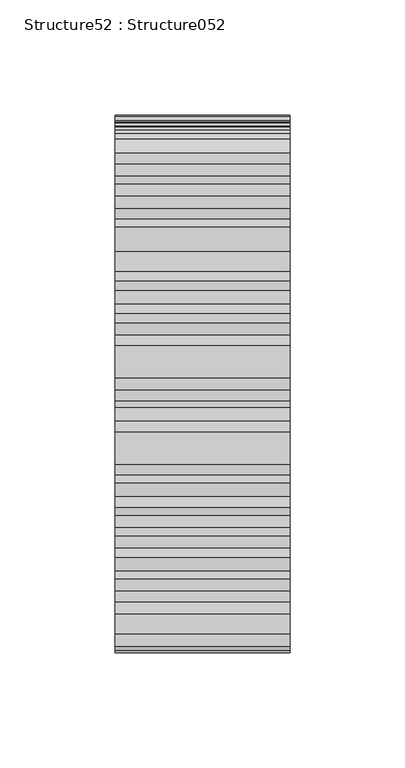
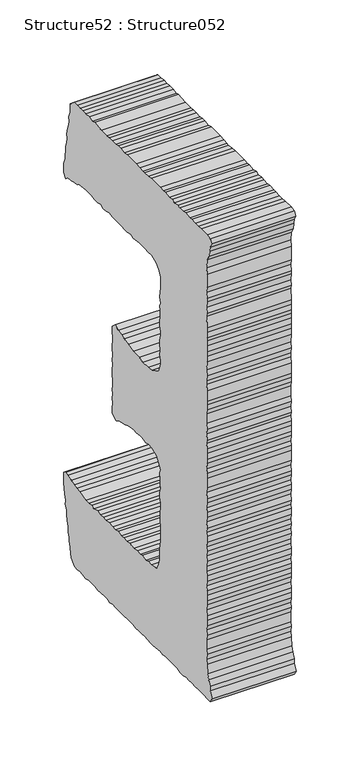
"""IFC4 building model written with IfcOpenShell, lengths in millimetres: proxy geometry, Structure52 : Structure052."""

import ifcopenshell
import ifcopenshell.guid

model = None  # the IFC model being written
_history = None  # IfcOwnerHistory: only IFC2X3 demands one
_inside = {}  # id of a spatial element -> (the spatial element, [elements in it])
_under = {}  # id of a project, library or spatial element -> (it, [spatial elements below it])
_declared = {}  # id of a project -> (the project, [libraries it declares])
_typed = {}  # id of a type object -> (the type object, [elements of that type])
_made_of = {}  # id of a material, layer set ... -> (it, [elements and type objects made of it])


def new_model(schema):
    """Start an empty IFC model of exactly this schema.

    Asked for "IFC4X3", IfcOpenShell would pick the latest addendum, in which some entities
    have other attributes; the version numbers below select the first issue.
    IFC2X3 requires an IfcOwnerHistory on every rooted entity: one is made here for all.
    """
    global model, _history
    if schema == "IFC4X3":
        model = ifcopenshell.file(schema_version=(4, 3, 0, 0))
    else:
        model = ifcopenshell.file(schema=schema)
    _inside.clear()
    _under.clear()
    _declared.clear()
    _typed.clear()
    _made_of.clear()
    _history = None
    if model.schema == "IFC2X3":
        org = make("IfcOrganization", Name="unknown")
        user = make(
            "IfcPersonAndOrganization",
            ThePerson=make("IfcPerson", FamilyName="unknown"),
            TheOrganization=org,
        )
        app = make(
            "IfcApplication",
            ApplicationDeveloper=org,
            Version="unknown",
            ApplicationFullName="unknown",
            ApplicationIdentifier="unknown",
        )
        _history = make(
            "IfcOwnerHistory",
            OwningUser=user,
            OwningApplication=app,
            ChangeAction="ADDED",
            CreationDate=0,
        )
    return model


def make(cls, **values):
    """One entity of the class cls with the attributes given. An attribute that is None is left unset."""
    return model.create_entity(
        cls, **{name: value for name, value in values.items() if value is not None}
    )


def rooted(cls, **values):
    """An entity with a GlobalId (a new one), such as an element, a storey or a relation."""
    return make(cls, GlobalId=ifcopenshell.guid.new(), OwnerHistory=_history, **values)


def si_unit(unit_type, name, prefix=None):
    """IfcSIUnit, for example si_unit("LENGTHUNIT", "METRE", prefix="MILLI")."""
    return make("IfcSIUnit", UnitType=unit_type, Prefix=prefix, Name=name)


def assignment(units):
    """IfcUnitAssignment: the units of a project."""
    return None if units is None else make("IfcUnitAssignment", Units=units)


def point(xyz):
    """IfcCartesianPoint."""
    return None if xyz is None else make("IfcCartesianPoint", Coordinates=xyz)


def direction(xyz):
    """IfcDirection."""
    return None if xyz is None else make("IfcDirection", DirectionRatios=xyz)


def frame(location, z_axis=None, x_axis=None):
    """IfcAxis2Placement3D, a coordinate frame: its origin and axes. An axis left out is left unset."""
    return make(
        "IfcAxis2Placement3D",
        Location=point(location),
        Axis=direction(z_axis),
        RefDirection=direction(x_axis),
    )


def origin():
    """The frame at (0, 0, 0) with its axes left unset."""
    return frame((0.0, 0.0, 0.0))


def place(relative_to, where):
    """IfcLocalPlacement: puts the frame where relative to a parent placement (None: the world)."""
    return make(
        "IfcLocalPlacement", PlacementRelTo=relative_to, RelativePlacement=where
    )


def context(
    kind, dimensions, precision=None, world=None, true_north=None, identifier=None
):
    """IfcGeometricRepresentationContext, for example the 3D "Model" context."""
    return make(
        "IfcGeometricRepresentationContext",
        ContextIdentifier=identifier,
        ContextType=kind,
        CoordinateSpaceDimension=dimensions,
        Precision=precision,
        WorldCoordinateSystem=world,
        TrueNorth=true_north,
    )


def project(units=None, contexts=None):
    """IfcProject with its units and contexts."""
    return rooted(
        "IfcProject",
        Name="project",
        RepresentationContexts=contexts,
        UnitsInContext=assignment(units),
    )


def spatial(cls, under=None, at=None, **own):
    """A site, building, storey or space (cls), placed at a placement, below another one or the project."""
    s = rooted(cls, ObjectPlacement=at, **own)
    if under is not None:
        _under.setdefault(under.id(), (under, []))[1].append(s)
    return s


def polyline(points):
    """IfcPolyline through the points."""
    return make("IfcPolyline", Points=[point(p) for p in points])


def outline(outer, holes=None, kind="AREA"):
    """IfcArbitraryClosedProfileDef: a profile drawn as a closed curve; with holes, ...WithVoids."""
    if holes is None:
        return make("IfcArbitraryClosedProfileDef", ProfileType=kind, OuterCurve=outer)
    return make(
        "IfcArbitraryProfileDefWithVoids",
        ProfileType=kind,
        OuterCurve=outer,
        InnerCurves=holes,
    )


def extrude(swept, where, along, depth):
    """IfcExtrudedAreaSolid: the profile swept, set in the frame where, extruded along a direction by depth."""
    return make(
        "IfcExtrudedAreaSolid",
        SweptArea=swept,
        Position=where,
        ExtrudedDirection=direction(along),
        Depth=depth,
    )


def shape(context_of_items, identifier, shape_type, items):
    """IfcShapeRepresentation: the items that make up one representation, for example the "Body"."""
    return make(
        "IfcShapeRepresentation",
        ContextOfItems=context_of_items,
        RepresentationIdentifier=identifier,
        RepresentationType=shape_type,
        Items=items,
    )


def source(mapping_origin, context_of_items, identifier, shape_type, items):
    """IfcRepresentationMap: a shape defined once, which mapped items show again and again."""
    return make(
        "IfcRepresentationMap",
        MappingOrigin=mapping_origin,
        MappedRepresentation=shape(context_of_items, identifier, shape_type, items),
    )


def transform(
    local_origin,
    x_axis=None,
    y_axis=None,
    z_axis=None,
    scale=None,
    scale2=None,
    scale3=None,
    uniform=True,
):
    """IfcCartesianTransformationOperator3D, or its non-uniform kind. x_axis, y_axis, z_axis: its Axis1, 2, 3."""
    if uniform:
        return make(
            "IfcCartesianTransformationOperator3D",
            Axis1=direction(x_axis),
            Axis2=direction(y_axis),
            LocalOrigin=point(local_origin),
            Scale=scale,
            Axis3=direction(z_axis),
        )
    return make(
        "IfcCartesianTransformationOperator3DnonUniform",
        Axis1=direction(x_axis),
        Axis2=direction(y_axis),
        LocalOrigin=point(local_origin),
        Scale=scale,
        Axis3=direction(z_axis),
        Scale2=scale2,
        Scale3=scale3,
    )


def mapped(mapping_source, mapping_target):
    """IfcMappedItem: shows the shape of a source again, moved by a transform."""
    return make(
        "IfcMappedItem", MappingSource=mapping_source, MappingTarget=mapping_target
    )


def made_of(thing, what):
    """Note that an element or type object is made of a material, layer set ...; save() writes the relation."""
    if what is not None:
        _made_of.setdefault(what.id(), (what, []))[1].append(thing)
    return thing


def element(
    cls,
    number,
    at=None,
    inside=None,
    cuts=None,
    type_object=None,
    material=None,
    context=None,
    identifier="Body",
    shape_type=None,
    held_by="IfcProductDefinitionShape",
    body=None,
    shapes=None,
    **own,
):
    """One element of the class cls, such as IfcWall. Its Tag is "e" and its number.

    at: its placement. inside: the storey or other place that contains it. cuts: it is an
    opening in that element (IfcRelVoidsElement). A single representation is given by context,
    identifier, shape_type and body (its items); several are given by shapes. held_by: the class
    of the entity that holds the representations. save() writes the other relations.
    """
    e = rooted(cls, Tag="e%d" % number, ObjectPlacement=at, **own)
    if body is not None:
        shapes = [shape(context, identifier, shape_type, body)]
    if shapes is not None:
        e.Representation = make(held_by, Representations=shapes)
    if inside is not None:
        _inside.setdefault(inside.id(), (inside, []))[1].append(e)
    if cuts is not None:
        rooted(
            "IfcRelVoidsElement", RelatingBuildingElement=cuts, RelatedOpeningElement=e
        )
    if type_object is not None:
        _typed.setdefault(type_object.id(), (type_object, []))[1].append(e)
    return made_of(e, material)


def aggregate(whole, parts):
    """IfcRelAggregates: a whole, such as a stair, and the parts it consists of."""
    return rooted("IfcRelAggregates", RelatingObject=whole, RelatedObjects=parts)


def save(model, path):
    """Write the relations noted so far, then the file.

    IfcRelAggregates (storeys below a building ...), IfcRelContainedInSpatialStructure (elements
    in a storey), IfcRelDefinesByType, IfcRelAssociatesMaterial and IfcRelDeclares: one each for
    every whole, place, type object, material and project.
    """
    for whole, parts in _under.values():
        aggregate(whole, parts)
    for where, things in _inside.values():
        rooted(
            "IfcRelContainedInSpatialStructure",
            RelatedElements=things,
            RelatingStructure=where,
        )
    for kind, things in _typed.values():
        rooted("IfcRelDefinesByType", RelatedObjects=things, RelatingType=kind)
    for what, things in _made_of.values():
        rooted("IfcRelAssociatesMaterial", RelatedObjects=things, RelatingMaterial=what)
    for by, libraries in _declared.values():
        rooted("IfcRelDeclares", RelatingContext=by, RelatedDefinitions=libraries)
    model.write(path)


def structure52_structure052_eb8b9618(model_context):
    return source(origin(), model_context, "Body", "SweptSolid", [
        extrude(outline(polyline([(256106.4891575, 3552.242032), (256102.9686552, 3551.0658569), (256097.6862972, 3551.6675836), (256088.3266392, 3550.4833855), (256084.2252701, 3551.6675836), (256073.6621587, 3551.6675836), (256070.1641209, 3550.4833855), (256064.3025007, 3551.0658569), (256059.5994049, 3551.6675836), (256054.9203782, 3551.6675836), (256050.8190091, 3550.4833855), (256046.1383778, 3551.6675836), (256041.4593511, 3551.0658569), (256027.3965973, 3551.0658569), (256023.8744904, 3551.6675836), (256014.4923679, 3551.6675836), (256009.2324744, 3550.4833855), (256005.1102455, 3551.0658569), (256000.4296141, 3551.0658569), (255995.1697206, 3551.6675836), (255991.6492183, 3551.0658569), (255986.3668603, 3550.4833855), (255982.2895603, 3550.4833855), (255971.7248443, 3551.6675836), (255967.6250798, 3551.0658569), (255962.9444485, 3551.6675836), (255944.7819302, 3551.6675836), (255940.0788345, 3550.4833855), (255935.3982031, 3550.4833855), (255930.696712, 3551.6675836), (255926.6178073, 3551.0658569), (255921.9387806, 3551.6675836), (255916.0546959, 3551.0658569), (255911.9533269, 3551.6675836), (255902.5936688, 3551.6675836), (255897.3113108, 3551.0658569), (255892.6098197, 3551.0658569), (255889.6894395, 3555.7416744), (255892.6098197, 3561.6257591), (255893.2115463, 3565.7094775), (255894.9717975, 3570.9854171), (255896.7320486, 3575.6853037), (255897.9130375, 3583.8864372), (255898.4922997, 3588.5702778), (255897.9130375, 3593.8285667), (255898.4922997, 3597.9540049), (255898.4922997, 3607.3393366), (255897.9130375, 3612.0135494), (255898.4922997, 3616.69739), (255897.3113108, 3621.3732075), (255897.3113108, 3626.6571701), (255897.9130375, 3630.7392839), (255898.4922997, 3636.0408972), (255897.9130375, 3641.2991861), (255897.3113108, 3645.4262289), (255897.9130375, 3650.1004418), (255897.3113108, 3654.7842823), (255898.4922997, 3658.8840468), (255897.9130375, 3663.5598643), (255897.9130375, 3668.8261762), (255898.4922997, 3672.9435914), (255898.4922997, 3677.6274319), (255897.9130375, 3682.8857208), (255898.4922997, 3687.587212), (255897.9130375, 3692.2710525), (255898.4922997, 3696.3884676), (255897.3113108, 3701.6547796), (255897.9130375, 3706.9130685), (255898.4922997, 3710.4560353), (255897.3113108, 3715.1302482), (255898.4922997, 3720.4158154), (255897.9130375, 3725.0996559), (255897.3113108, 3730.3563402), (255898.4922997, 3733.8736333), (255897.9130375, 3739.1592005), (255897.3113108, 3743.2332913), (255898.4922997, 3748.5429276), (255897.9130375, 3753.2171405), (255897.9130375, 3762.5848215), (255897.3113108, 3767.8607611), (255898.4922997, 3771.3860772), (255897.3113108, 3777.2444882), (255897.3113108, 3781.3282066), (255897.9130375, 3786.6298199), (255897.3113108, 3791.3056374), (255898.4922997, 3795.960595), (255897.3113108, 3799.5051664), (255898.4922997, 3804.7730829), (255897.3113108, 3810.0474179), (255898.4922997, 3814.7296538), (255898.4922997, 3824.1149855), (255897.9130375, 3828.2163546), (255897.9130375, 3832.8921721), (255897.3113108, 3836.9919366), (255897.3113108, 3846.9757858), (255898.4922997, 3852.2340747), (255898.4922997, 3855.7353217), (255897.9130375, 3861.0192843), (255898.4922997, 3866.3032469), (255897.3113108, 3874.5043805), (255897.9130375, 3879.7610648), (255897.3113108, 3884.4609514), (255897.9130375, 3889.7208449), (255897.9130375, 3894.4030808), (255897.3113108, 3897.9476522), (255897.9130375, 3902.6314927), (255897.3113108, 3907.3313793), (255898.4922997, 3917.8479571), (255897.3113108, 3921.3748778), (255898.4922997, 3926.0490907), (255897.9130375, 3931.9058971), (255897.3113108, 3935.4328178), (255898.4922997, 3940.718385), (255897.3113108, 3945.9766739), (255897.3113108, 3958.8776941), (255898.4922997, 3964.1343784), (255897.3113108, 3972.3627903), (255894.3700708, 3977.6194746), (255893.7908086, 3982.8793681), (255892.6098197, 3987.5792547), (255890.8704284, 3991.6806238), (255892.6098197, 3995.7803883), (255897.9130375, 3996.390138), (255906.6950379, 3996.390138), (255911.9533269, 3995.7803883), (255916.6339582, 3995.7803883), (255921.9387806, 3996.390138), (255925.4368184, 3995.7803883), (255931.2984387, 3996.9645864), (255935.3982031, 3995.7803883), (255940.6805611, 3996.390138), (255944.202668, 3996.390138), (255949.4609569, 3995.7803883), (255952.9605993, 3996.9645864), (255957.6620905, 3995.7803883), (255963.5237107, 3996.9645864), (255967.0458176, 3996.390138), (255971.7248443, 3996.9645864), (255985.7875981, 3996.9645864), (255990.4682294, 3996.390138), (255996.3523141, 3995.7803883), (255999.2486252, 3995.7803883), (256003.951721, 3996.390138), (256009.2324744, 3996.9645864), (256023.2952282, 3996.9645864), (256027.9758595, 3995.7803883), (256033.2582175, 3996.9645864), (256037.3355175, 3996.9645864), (256041.4593511, 3995.7803883), (256047.3193667, 3995.7803883), (256051.3982713, 3996.390138), (256055.5221049, 3995.7803883), (256064.3025007, 3995.7803883), (256074.8431476, 3996.9645864), (256078.3652545, 3995.7803883), (256083.0442812, 3996.9645864), (256088.3266392, 3996.9645864), (256093.6089972, 3996.390138), (256097.107035, 3996.9645864), (256102.389393, 3996.390138), (256107.0700243, 3996.390138), (256112.9300399, 3991.6806238), (256112.9300399, 3988.1633307), (256112.9300399, 3983.4794902), (256115.2711579, 3977.6194746), (256114.6918957, 3973.5197101), (256115.2711579, 3969.994394), (256117.0538735, 3965.3201811), (256118.1899335, 3959.4617701), (256117.6106712, 3955.360401), (256118.7916602, 3951.2606365), (256119.9501846, 3946.5511223), (256119.9501846, 3942.4770315), (256120.5519113, 3937.1930689), (256121.1311735, 3933.6741713), (256122.8930292, 3928.4158823), (256123.4947559, 3924.2888396), (256123.4947559, 3919.6066036), (256119.9501846, 3915.5068392), (256117.0538735, 3917.8479571), (256111.749051, 3918.4480792), (256107.0700243, 3919.6066036), (256102.389393, 3920.2067257), (256099.4690128, 3922.5494483), (256088.9059014, 3923.7079727), (256079.5462434, 3923.7079727), (256075.4224098, 3922.5494483), (256070.1641209, 3922.5494483), (256065.4610251, 3923.7079727), (256060.7803938, 3922.5494483), (256056.7030938, 3922.5494483), (256051.999998, 3923.7079727), (256046.1383778, 3923.1319197), (256032.075624, 3923.1319197), (256027.3965973, 3922.5494483), (256023.2952282, 3922.5494483), (256018.0144748, 3923.7079727), (256013.9131057, 3922.5494483), (256008.0514855, 3923.1319197), (256004.5534477, 3923.7079727), (255995.1697206, 3923.7079727), (255990.4682294, 3923.1319197), (255985.2083359, 3923.7079727), (255977.5864645, 3920.7908018), (255974.0884267, 3916.6653636), (255971.1455821, 3910.8310217), (255971.1455821, 3900.2887701), (255971.7248443, 3896.763454), (255972.3041065, 3891.5067697), (255971.1455821, 3886.2051565), (255972.3041065, 3883.2863809), (255971.7248443, 3878.5784713), (255971.7248443, 3873.3185778), (255972.3041065, 3868.0618934), (255972.3041065, 3863.9332461), (255971.1455821, 3859.2606378), (255971.1455821, 3855.1769193), (255972.3041065, 3849.8753061), (255972.3041065, 3845.8012153), (255971.7248443, 3840.5172527), (255972.3041065, 3835.8334121), (255971.1455821, 3831.1575946), (255971.1455821, 3827.6162325), (255974.0884267, 3818.8310229), (255984.6066092, 3813.5743386), (255990.4682294, 3812.9726119), (255998.669363, 3812.9726119), (256004.5534477, 3814.148787), (256013.9131057, 3814.148787), (256022.1142393, 3815.9154565), (256027.9758595, 3817.6741031), (256032.075624, 3818.8310229), (256037.3355175, 3820.015221), (256042.0386133, 3822.348316), (256046.71764, 3818.2309008), (256047.3193667, 3814.7296538), (256046.1383778, 3805.3459267), (256046.71764, 3799.5051664), (256047.3193667, 3795.960595), (256046.1383778, 3791.3056374), (256046.71764, 3785.4456218), (256046.1383778, 3781.9299333), (256047.3193667, 3776.6427615), (256047.3193667, 3771.3860772), (256046.1383778, 3766.684586), (256046.1383778, 3762.0023501), (256046.71764, 3757.8753073), (256046.1383778, 3753.8012165), (256047.3193667, 3748.5429276), (256046.1383778, 3744.4158848), (256046.71764, 3739.7416719), (256046.71764, 3734.47536), (256040.8800889, 3730.9323932), (256036.7562553, 3733.2991849), (256032.6564908, 3734.47536), (256026.8173351, 3735.6146291), (256022.1142393, 3737.400554), (256013.311379, 3739.1592005), (256009.2324744, 3738.5574738), (256003.3724588, 3739.1592005), (255999.8503519, 3739.7416719), (255993.9887317, 3738.5574738), (255989.9114317, 3739.1592005), (255984.6066092, 3739.1592005), (255976.9847379, 3736.2163558), (255975.2244867, 3733.8736333), (255971.1455821, 3726.2742264), (255972.3041065, 3722.7312597), (255971.7248443, 3716.8985223), (255971.7248443, 3712.2146818), (255971.1455821, 3708.087639), (255972.3041065, 3704.0135482), (255972.3041065, 3699.3136616), (255971.1455821, 3694.029699), (255971.1455821, 3689.3458585), (255971.7248443, 3685.8285655), (255971.7248443, 3677.0449605), (255971.1455821, 3671.7690209), (255971.1455821, 3657.7014533), (255971.7248443, 3654.1841602), (255972.3041065, 3648.9258713), (255972.3041065, 3638.9580681), (255974.667689, 3631.915459), (255976.9847379, 3628.4158166), (255985.7875981, 3626.0554434), (255990.4682294, 3626.6571701), (255993.9887317, 3625.472972), (255999.8503519, 3626.6571701), (256003.3724588, 3625.472972), (256008.0514855, 3626.0554434), (256013.311379, 3625.472972), (256019.1954637, 3626.6571701), (256023.8744904, 3625.472972), (256028.5551217, 3626.0554434), (256032.6564908, 3625.472972), (256037.9372442, 3626.6571701), (256042.0386133, 3625.472972), (256046.1383778, 3626.0554434), (256051.3982713, 3626.6571701), (256057.282356, 3625.472972), (256061.3821205, 3626.0554434), (256066.0402874, 3625.472972), (256070.1641209, 3626.6571701), (256076.0241365, 3625.472972), (256079.5462434, 3626.6571701), (256084.2252701, 3625.472972), (256088.9059014, 3625.472972), (256098.2880239, 3627.8397636), (256102.9686552, 3628.4158166), (256107.0700243, 3629.5984101), (256111.1697888, 3631.3410106), (256117.0538735, 3632.5155811), (256119.9501846, 3633.6821286), (256123.4947559, 3631.3410106), (256123.4947559, 3625.472972), (256123.4947559, 3620.7971545), (256122.313767, 3617.2718384), (256121.7329002, 3611.4134274), (256119.9501846, 3606.7295868), (256120.5519113, 3602.6298224), (256118.1899335, 3598.5284533), (256118.7916602, 3593.8285667), (256117.6106712, 3588.5702778), (256115.8728846, 3584.4689087), (256115.8728846, 3578.6104977), (256114.6918957, 3574.5107332), (256114.6918957, 3570.4109687), (256112.9300399, 3565.7094775), (256112.3507777, 3559.8671125), (256111.749051, 3556.3417965), (256106.4891575, 3552.242032)])), frame((-38594.2176606, 0.0, 0.0), z_axis=(1.0, 0.0, 0.0), x_axis=(0.0, 1.0, 0.0)), (0.0, 0.0, 1.0), 76.2),
    ])


if __name__ == "__main__":
    model = new_model("IFC4")
    model_context = context("Model", 3, world=origin())
    ifc_project = project(units=[si_unit("LENGTHUNIT", "METRE", prefix="MILLI")], contexts=[model_context])
    site = spatial("IfcSite", under=ifc_project)
    building = spatial("IfcBuilding", under=site)
    placement = place(None, origin())
    structure52_structure052_shape = structure52_structure052_eb8b9618(model_context)
    element("IfcBuildingElementProxy", 1, Name="Structure52 : Structure052", ObjectType="Structure52 : Structure052", at=placement, inside=building, context=model_context, shape_type="MappedRepresentation", body=[
        mapped(structure52_structure052_shape, transform((0.0, 0.0, 0.0), x_axis=(1.0, 0.0, 0.0), y_axis=(0.0, 1.0, 0.0), z_axis=(0.0, 0.0, 1.0))),
    ])
    save(model, "model.ifc")

# Revit data of these elements
# Type "Structure52 : Structure052"
#   NameOverride = "Structure052"
# Element 1 (IfcBuildingElementProxy, "Structure52 : Structure052")
#   Materials on its faces: "BRUSHED ALUM. LETTERING"
# Materials
#   "BRUSHED ALUM. LETTERING": class "Unassigned", colour RGB 169 181 186, transparency 0, Cost = 0
